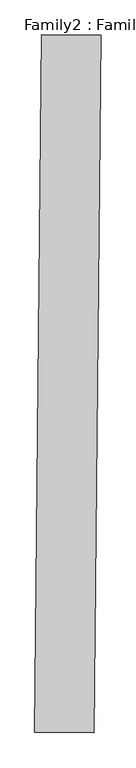
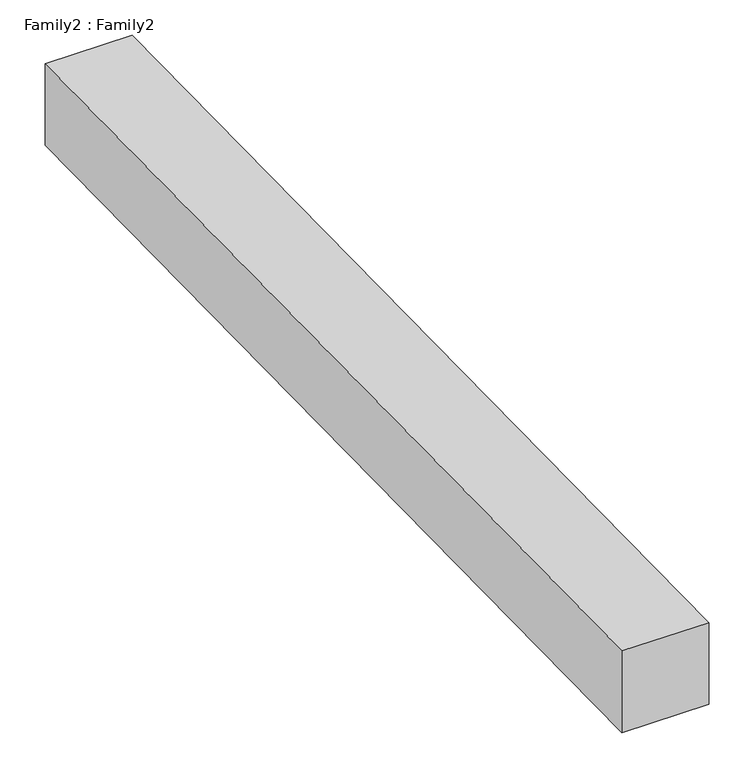
"""IFC4 building model written with IfcOpenShell, lengths in millimetres: proxy geometry, Family2 : Family2."""

import ifcopenshell
import ifcopenshell.guid

model = None  # the IFC model being written
_history = None  # IfcOwnerHistory: only IFC2X3 demands one
_inside = {}  # id of a spatial element -> (the spatial element, [elements in it])
_under = {}  # id of a project, library or spatial element -> (it, [spatial elements below it])
_declared = {}  # id of a project -> (the project, [libraries it declares])
_typed = {}  # id of a type object -> (the type object, [elements of that type])
_made_of = {}  # id of a material, layer set ... -> (it, [elements and type objects made of it])


def new_model(schema):
    """Start an empty IFC model of exactly this schema.

    Asked for "IFC4X3", IfcOpenShell would pick the latest addendum, in which some entities
    have other attributes; the version numbers below select the first issue.
    IFC2X3 requires an IfcOwnerHistory on every rooted entity: one is made here for all.
    """
    global model, _history
    if schema == "IFC4X3":
        model = ifcopenshell.file(schema_version=(4, 3, 0, 0))
    else:
        model = ifcopenshell.file(schema=schema)
    _inside.clear()
    _under.clear()
    _declared.clear()
    _typed.clear()
    _made_of.clear()
    _history = None
    if model.schema == "IFC2X3":
        org = make("IfcOrganization", Name="unknown")
        user = make(
            "IfcPersonAndOrganization",
            ThePerson=make("IfcPerson", FamilyName="unknown"),
            TheOrganization=org,
        )
        app = make(
            "IfcApplication",
            ApplicationDeveloper=org,
            Version="unknown",
            ApplicationFullName="unknown",
            ApplicationIdentifier="unknown",
        )
        _history = make(
            "IfcOwnerHistory",
            OwningUser=user,
            OwningApplication=app,
            ChangeAction="ADDED",
            CreationDate=0,
        )
    return model


def make(cls, **values):
    """One entity of the class cls with the attributes given. An attribute that is None is left unset."""
    return model.create_entity(
        cls, **{name: value for name, value in values.items() if value is not None}
    )


def rooted(cls, **values):
    """An entity with a GlobalId (a new one), such as an element, a storey or a relation."""
    return make(cls, GlobalId=ifcopenshell.guid.new(), OwnerHistory=_history, **values)


def si_unit(unit_type, name, prefix=None):
    """IfcSIUnit, for example si_unit("LENGTHUNIT", "METRE", prefix="MILLI")."""
    return make("IfcSIUnit", UnitType=unit_type, Prefix=prefix, Name=name)


def assignment(units):
    """IfcUnitAssignment: the units of a project."""
    return None if units is None else make("IfcUnitAssignment", Units=units)


def point(xyz):
    """IfcCartesianPoint."""
    return None if xyz is None else make("IfcCartesianPoint", Coordinates=xyz)


def direction(xyz):
    """IfcDirection."""
    return None if xyz is None else make("IfcDirection", DirectionRatios=xyz)


def frame(location, z_axis=None, x_axis=None):
    """IfcAxis2Placement3D, a coordinate frame: its origin and axes. An axis left out is left unset."""
    return make(
        "IfcAxis2Placement3D",
        Location=point(location),
        Axis=direction(z_axis),
        RefDirection=direction(x_axis),
    )


def origin():
    """The frame at (0, 0, 0) with its axes left unset."""
    return frame((0.0, 0.0, 0.0))


def place(relative_to, where):
    """IfcLocalPlacement: puts the frame where relative to a parent placement (None: the world)."""
    return make(
        "IfcLocalPlacement", PlacementRelTo=relative_to, RelativePlacement=where
    )


def context(
    kind, dimensions, precision=None, world=None, true_north=None, identifier=None
):
    """IfcGeometricRepresentationContext, for example the 3D "Model" context."""
    return make(
        "IfcGeometricRepresentationContext",
        ContextIdentifier=identifier,
        ContextType=kind,
        CoordinateSpaceDimension=dimensions,
        Precision=precision,
        WorldCoordinateSystem=world,
        TrueNorth=true_north,
    )


def project(units=None, contexts=None):
    """IfcProject with its units and contexts."""
    return rooted(
        "IfcProject",
        Name="project",
        RepresentationContexts=contexts,
        UnitsInContext=assignment(units),
    )


def spatial(cls, under=None, at=None, **own):
    """A site, building, storey or space (cls), placed at a placement, below another one or the project."""
    s = rooted(cls, ObjectPlacement=at, **own)
    if under is not None:
        _under.setdefault(under.id(), (under, []))[1].append(s)
    return s


def faces_of(points, faces, orient=None, outer=None):
    """IfcFace entities. A face is a list of loops; a loop is a list of indices into points, from 0.

    orient and outer hold one flag for each loop. By default every Orientation is true, the
    first loop of a face is its IfcFaceOuterBound and the others are IfcFaceBound.
    """
    made = []
    for i, loops in enumerate(faces):
        bounds = []
        for j, loop in enumerate(loops):
            is_outer = j == 0 if outer is None else outer[i][j]
            bounds.append(
                make(
                    "IfcFaceOuterBound" if is_outer else "IfcFaceBound",
                    Bound=make("IfcPolyLoop", Polygon=[points[k] for k in loop]),
                    Orientation=True if orient is None else orient[i][j],
                )
            )
        made.append(make("IfcFace", Bounds=bounds))
    return made


def faceted_brep(points, faces, orient=None, outer=None, voids=None):
    """IfcFacetedBrep: a solid bounded by flat faces; with voids (closed shells), ...WithVoids."""
    shared = [point(p) for p in points]
    hull = make("IfcClosedShell", CfsFaces=faces_of(shared, faces, orient, outer))
    if voids is None:
        return make("IfcFacetedBrep", Outer=hull)
    return make(
        "IfcFacetedBrepWithVoids",
        Outer=hull,
        Voids=[
            make(cls, CfsFaces=faces_of(shared, fs, o, b)) for cls, fs, o, b in voids
        ],
    )


def shape(context_of_items, identifier, shape_type, items):
    """IfcShapeRepresentation: the items that make up one representation, for example the "Body"."""
    return make(
        "IfcShapeRepresentation",
        ContextOfItems=context_of_items,
        RepresentationIdentifier=identifier,
        RepresentationType=shape_type,
        Items=items,
    )


def source(mapping_origin, context_of_items, identifier, shape_type, items):
    """IfcRepresentationMap: a shape defined once, which mapped items show again and again."""
    return make(
        "IfcRepresentationMap",
        MappingOrigin=mapping_origin,
        MappedRepresentation=shape(context_of_items, identifier, shape_type, items),
    )


def transform(
    local_origin,
    x_axis=None,
    y_axis=None,
    z_axis=None,
    scale=None,
    scale2=None,
    scale3=None,
    uniform=True,
):
    """IfcCartesianTransformationOperator3D, or its non-uniform kind. x_axis, y_axis, z_axis: its Axis1, 2, 3."""
    if uniform:
        return make(
            "IfcCartesianTransformationOperator3D",
            Axis1=direction(x_axis),
            Axis2=direction(y_axis),
            LocalOrigin=point(local_origin),
            Scale=scale,
            Axis3=direction(z_axis),
        )
    return make(
        "IfcCartesianTransformationOperator3DnonUniform",
        Axis1=direction(x_axis),
        Axis2=direction(y_axis),
        LocalOrigin=point(local_origin),
        Scale=scale,
        Axis3=direction(z_axis),
        Scale2=scale2,
        Scale3=scale3,
    )


def mapped(mapping_source, mapping_target):
    """IfcMappedItem: shows the shape of a source again, moved by a transform."""
    return make(
        "IfcMappedItem", MappingSource=mapping_source, MappingTarget=mapping_target
    )


def made_of(thing, what):
    """Note that an element or type object is made of a material, layer set ...; save() writes the relation."""
    if what is not None:
        _made_of.setdefault(what.id(), (what, []))[1].append(thing)
    return thing


def element(
    cls,
    number,
    at=None,
    inside=None,
    cuts=None,
    type_object=None,
    material=None,
    context=None,
    identifier="Body",
    shape_type=None,
    held_by="IfcProductDefinitionShape",
    body=None,
    shapes=None,
    **own,
):
    """One element of the class cls, such as IfcWall. Its Tag is "e" and its number.

    at: its placement. inside: the storey or other place that contains it. cuts: it is an
    opening in that element (IfcRelVoidsElement). A single representation is given by context,
    identifier, shape_type and body (its items); several are given by shapes. held_by: the class
    of the entity that holds the representations. save() writes the other relations.
    """
    e = rooted(cls, Tag="e%d" % number, ObjectPlacement=at, **own)
    if body is not None:
        shapes = [shape(context, identifier, shape_type, body)]
    if shapes is not None:
        e.Representation = make(held_by, Representations=shapes)
    if inside is not None:
        _inside.setdefault(inside.id(), (inside, []))[1].append(e)
    if cuts is not None:
        rooted(
            "IfcRelVoidsElement", RelatingBuildingElement=cuts, RelatedOpeningElement=e
        )
    if type_object is not None:
        _typed.setdefault(type_object.id(), (type_object, []))[1].append(e)
    return made_of(e, material)


def aggregate(whole, parts):
    """IfcRelAggregates: a whole, such as a stair, and the parts it consists of."""
    return rooted("IfcRelAggregates", RelatingObject=whole, RelatedObjects=parts)


def save(model, path):
    """Write the relations noted so far, then the file.

    IfcRelAggregates (storeys below a building ...), IfcRelContainedInSpatialStructure (elements
    in a storey), IfcRelDefinesByType, IfcRelAssociatesMaterial and IfcRelDeclares: one each for
    every whole, place, type object, material and project.
    """
    for whole, parts in _under.values():
        aggregate(whole, parts)
    for where, things in _inside.values():
        rooted(
            "IfcRelContainedInSpatialStructure",
            RelatedElements=things,
            RelatingStructure=where,
        )
    for kind, things in _typed.values():
        rooted("IfcRelDefinesByType", RelatedObjects=things, RelatingType=kind)
    for what, things in _made_of.values():
        rooted("IfcRelAssociatesMaterial", RelatedObjects=things, RelatingMaterial=what)
    for by, libraries in _declared.values():
        rooted("IfcRelDeclares", RelatingContext=by, RelatedDefinitions=libraries)
    model.write(path)


def family2_family2_bd8c0e6c(model_context):
    return source(origin(), model_context, "Body", "Brep", [
        faceted_brep([(-3955.2766933, -7250.0373466, 1.0945136), (-3955.2766933, -7250.0373466, 201.0945136), (-3931.5661012, -4897.5627761, 202.060409), (-3931.5661012, -4897.5627761, 2.060409), (-3755.2855033, -7251.9145592, 201.0945136), (-3731.5749112, -4899.4399887, 202.060409), (-3755.2855033, -7251.9145592, 1.0945136), (-3731.5749112, -4899.4399887, 2.060409)], [[[0, 1, 2, 3]], [[1, 4, 5, 2]], [[4, 6, 7, 5]], [[6, 0, 3, 7]], [[3, 2, 5, 7]], [[0, 6, 4, 1]]]),
    ])


if __name__ == "__main__":
    model = new_model("IFC4")
    model_context = context("Model", 3, world=origin())
    ifc_project = project(units=[si_unit("LENGTHUNIT", "METRE", prefix="MILLI")], contexts=[model_context])
    site = spatial("IfcSite", under=ifc_project)
    building = spatial("IfcBuilding", under=site)
    placement = place(None, origin())
    family2_family2_shape = family2_family2_bd8c0e6c(model_context)
    element("IfcBuildingElementProxy", 1, Name="Family2 : Family2", ObjectType="Family2 : Family2", at=placement, inside=building, context=model_context, shape_type="MappedRepresentation", body=[
        mapped(family2_family2_shape, transform((0.0, 0.0, 0.0), x_axis=(1.0, 0.0, 0.0), y_axis=(0.0, 1.0, 0.0), z_axis=(0.0, 0.0, 1.0))),
    ])
    save(model, "model.ifc")

# Revit data of these elements
# Type "Family2 : Family2"
#   Default Elevation = 0
